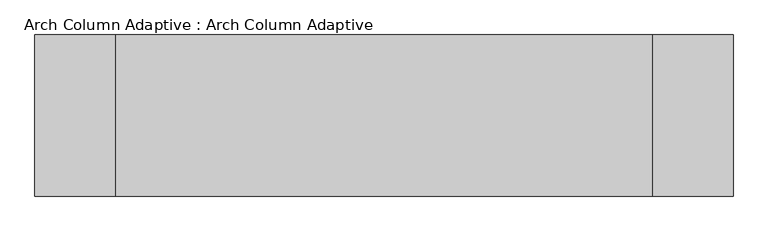
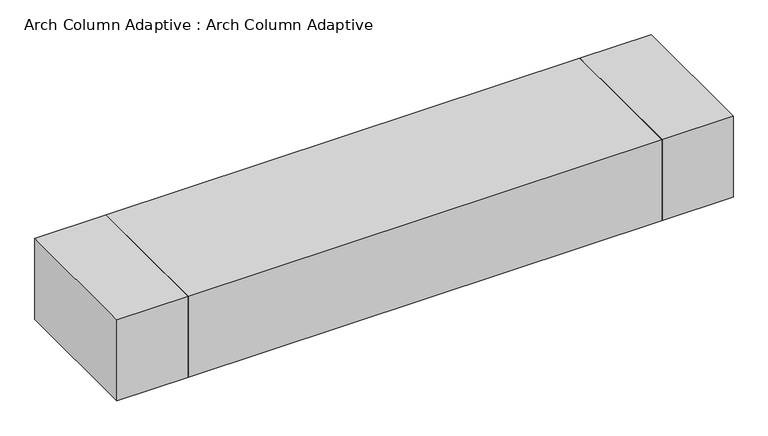
"""IFC4 building model written with IfcOpenShell, lengths in millimetres: proxy geometry, Arch Column Adaptive : Arch Column Adaptive."""

from ifc_helpers import new_model, si_unit, frame, origin, place, context, project, spatial, polyline, outline, extrude, source, transform, mapped, element, save


def arch_column_adaptive_arch_column_adaptive_599e5d12(model_context):
    return source(origin(), model_context, "Body", "SweptSolid", [
        extrude(outline(polyline([(5000.0, -1500.0), (5000.0, 1500.0), (6500.0, 1500.0), (6500.0, -1500.0), (5000.0, -1500.0)])), frame((0.0, 0.0, 7047.5), z_axis=(0.0, 0.0, 1.0), x_axis=(1.0, 0.0, 0.0)), (0.0, 0.0, 1.0), 1800.0),
        extrude(outline(polyline([(-5000.0, 1500.0), (-5000.0, -1500.0), (-6500.0, -1500.0), (-6500.0, 1500.0), (-5000.0, 1500.0)])), frame((0.0, 0.0, 7047.5), z_axis=(0.0, 0.0, 1.0), x_axis=(1.0, 0.0, 0.0)), (0.0, 0.0, 1.0), 1800.0),
        extrude(outline(polyline([(-5000.0, -1500.0), (-5000.0, 1500.0), (5000.0, 1500.0), (5000.0, -1500.0), (-5000.0, -1500.0)])), frame((0.0, 0.0, 7047.5), z_axis=(0.0, 0.0, 1.0), x_axis=(1.0, 0.0, 0.0)), (0.0, 0.0, 1.0), 1800.0),
    ])


if __name__ == "__main__":
    model = new_model("IFC4")
    model_context = context("Model", 3, world=origin())
    ifc_project = project(units=[si_unit("LENGTHUNIT", "METRE", prefix="MILLI")], contexts=[model_context])
    site = spatial("IfcSite", under=ifc_project)
    building = spatial("IfcBuilding", under=site)
    placement = place(None, origin())
    arch_column_adaptive_arch_column_adaptive_shape = arch_column_adaptive_arch_column_adaptive_599e5d12(model_context)
    element("IfcBuildingElementProxy", 1, Name="Arch Column Adaptive : Arch Column Adaptive", ObjectType="Arch Column Adaptive : Arch Column Adaptive", at=placement, inside=building, context=model_context, shape_type="MappedRepresentation", body=[
        mapped(arch_column_adaptive_arch_column_adaptive_shape, transform((0.0, 0.0, 0.0), x_axis=(1.0, 0.0, 0.0), y_axis=(0.0, 1.0, 0.0), z_axis=(0.0, 0.0, 1.0))),
    ])
    save(model, "model.ifc")

# Revit data of these elements
# Type "Arch Column Adaptive : Arch Column Adaptive"
#   Top Width = 3000 mm
#   Length [instance default] = 21000 mm
#   Height [instance default] = 50000 mm
#   Default Elevation = 0
# Element 1 (IfcBuildingElementProxy, "Arch Column Adaptive : Arch Column Adaptive")
#   Height = 7047.5 mm
